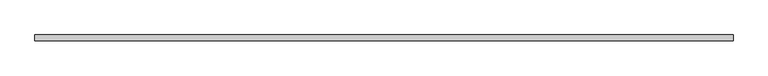
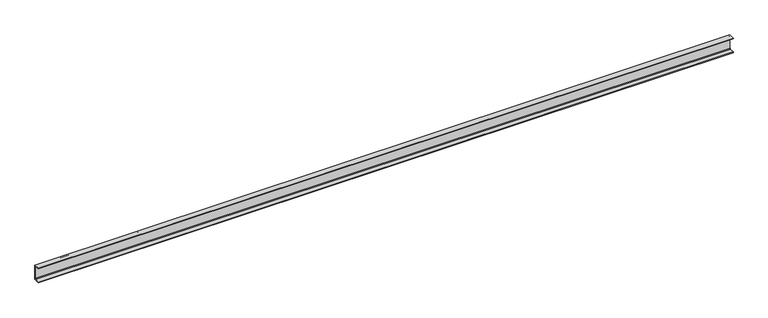
"""IFC4 building model written with IfcOpenShell, lengths in millimetres: beam geometry, С-образный профиль с параллельными полками (ГОСТ 8240-89) Балки : [ 20P."""

from ifc_helpers import new_model, si_unit, point, frame, frame_2d, origin, place, context, project, spatial, polyline, circle_curve, trimmed, segment, composite_curve, outline, extrude, source, transform, mapped, element, save


def beam_e8fb0e59(model_context):
    return source(origin(), model_context, "Body", "SweptSolid", [
        extrude(outline(composite_curve([segment(polyline([(23.0, 100.0), (23.0, -100.0), (-53.0, -100.0), (-53.0, -91.0), (8.3, -91.0)]), True, "CONTINUOUS"), segment(trimmed(circle_curve(frame_2d((8.3, -81.5)), 9.5), [point((8.3, -91.0))], [point((17.8, -81.5))], True, "CARTESIAN"), True, "CONTINUOUS"), segment(polyline([(17.8, -81.5), (17.8, 81.5)]), True, "CONTINUOUS"), segment(trimmed(circle_curve(frame_2d((8.3, 81.5)), 9.5), [point((17.8, 81.5))], [point((8.3, 91.0))], True, "CARTESIAN"), True, "CONTINUOUS"), segment(polyline([(8.3, 91.0), (-53.0, 91.0), (-53.0, 100.0), (23.0, 100.0)]), True, "CONTINUOUS")], self_intersect=False)), frame((-4585.0, 0.0, 0.0), z_axis=(1.0, 0.0, 0.0), x_axis=(0.0, 1.0, 0.0)), (0.0, 0.0, 1.0), 9170.0),
    ])


if __name__ == "__main__":
    model = new_model("IFC4")
    model_context = context("Model", 3, world=origin())
    ifc_project = project(units=[si_unit("LENGTHUNIT", "METRE", prefix="MILLI")], contexts=[model_context])
    site = spatial("IfcSite", under=ifc_project)
    building = spatial("IfcBuilding", under=site)
    placement = place(None, origin())
    beam_shape = beam_e8fb0e59(model_context)
    element("IfcBeam", 1, ObjectType="С-образный профиль с параллельными полками (ГОСТ 8240-89) Балки : [ 20P", at=placement, inside=building, context=model_context, shape_type="MappedRepresentation", body=[
        mapped(beam_shape, transform((0.0, 0.0, 0.0), x_axis=(1.0, 0.0, 0.0), y_axis=(0.0, 1.0, 0.0), z_axis=(0.0, 0.0, 1.0))),
    ])
    save(model, "model.ifc")

# Revit data of these elements
# Type "С-образный профиль с параллельными полками (ГОСТ 8240-89) Балки : [ 20P"
#   tf = 9 mm
#   ra = 9.5 mm
#   W = 0.180442
#   Vz = 100 mm
#   Vy = 53 mm
#   Vpz = 100 mm
#   Vpy = 23 mm
#   Length [instance default] = 1500 mm
#   bf = 76 mm
#   d = 200 mm
#   tw = 5.2 mm
#   A = 0.00234 m²
#   Structural Material [instance default] = Металл - Сталь - 345 МПa
#   Assembly Code = ""
# Element 1 (IfcBeam, "С-образный профиль с параллельными полками (ГОСТ 8240-89) Балки : [ 20P")
#   Structural Material = C245
#   Materials on its faces: "C245"
# Materials
#   "Металл - Сталь - 345 МПa": class "Металл", colour RGB 247 247 247, transparency 0
#   "C245": class "Не назначено", colour RGB 0 0 0, transparency 0
